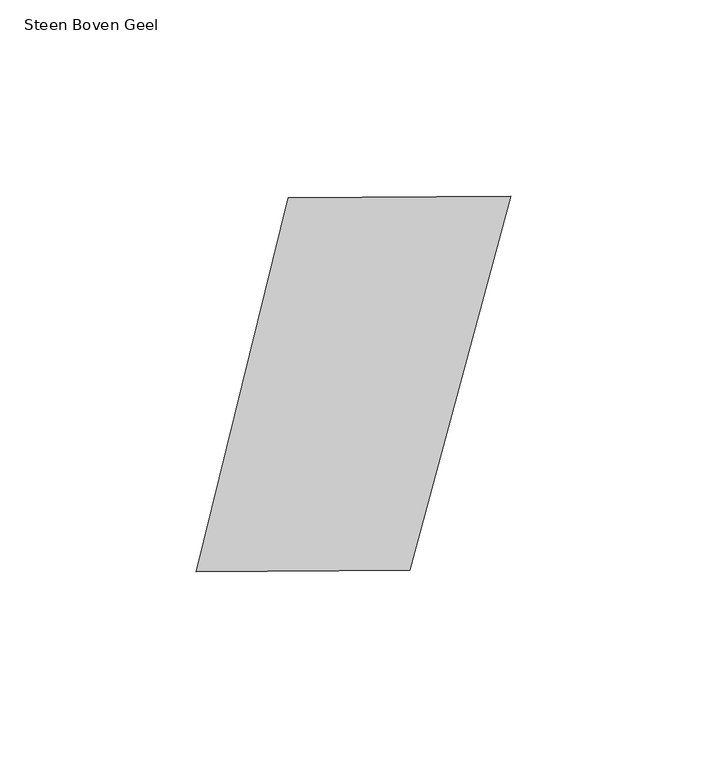
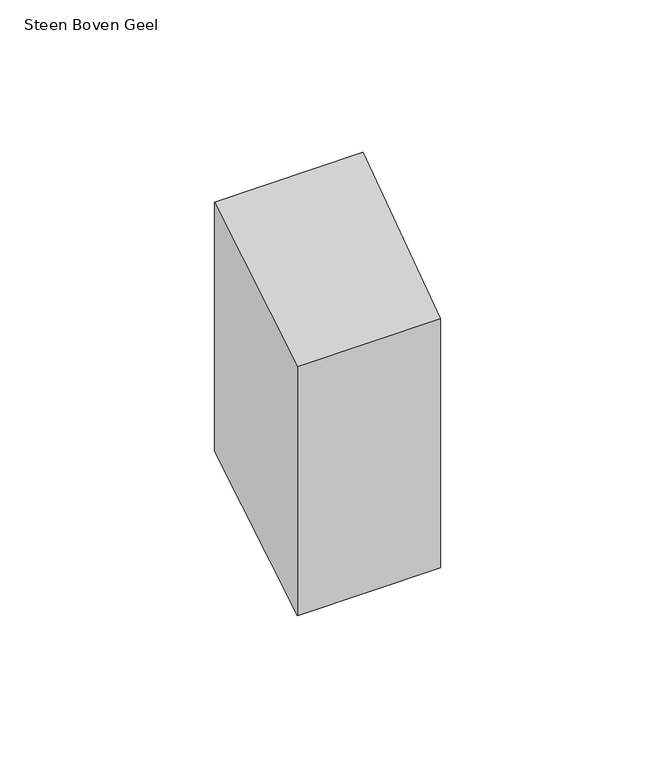
"""IFC4 building model written with IfcOpenShell, lengths in millimetres: proxy geometry, 00_GMA_steen_versie_4 : Steen Boven Geel."""

from ifc_helpers import new_model, si_unit, origin, origin_with_axes, place, context, project, spatial, polyline, outline, extrude, source, transform, mapped, element, save


def steen_boven_geel_e52851ac(model_context):
    return source(origin(), model_context, "Body", "SweptSolid", [
        extrude(outline(polyline([(114.0326098, 118.6673556), (88.372725, 23.2738668), (33.8296928, 22.8501526), (57.3678401, 118.2036955), (114.0326098, 118.6673556)])), origin_with_axes(), (0.0, 0.0, 1.0), 100.0),
    ])


if __name__ == "__main__":
    model = new_model("IFC4")
    model_context = context("Model", 3, world=origin())
    ifc_project = project(units=[si_unit("LENGTHUNIT", "METRE", prefix="MILLI")], contexts=[model_context])
    site = spatial("IfcSite", under=ifc_project)
    building = spatial("IfcBuilding", under=site)
    placement = place(None, origin())
    steen_boven_geel_shape = steen_boven_geel_e52851ac(model_context)
    element("IfcBuildingElementProxy", 1, Name="00_GMA_steen_versie_4 : Steen Boven Geel", ObjectType="00_GMA_steen_versie_4 : Steen Boven Geel", at=placement, inside=building, context=model_context, shape_type="MappedRepresentation", body=[
        mapped(steen_boven_geel_shape, transform((0.0, 0.0, 0.0), x_axis=(1.0, 0.0, 0.0), y_axis=(0.0, 1.0, 0.0), z_axis=(0.0, 0.0, 1.0))),
    ])
    save(model, "model.ifc")

# Revit data of these elements
# Type "00_GMA_steen_versie_4 : Steen Boven Geel"
#   StootVoegHalfBoven [instance default] = 5 mm
#   StootVoegHalf [instance default] = 5 mm
#   StootVoegBreedteOnder = 10 mm
#   StootVoegBreedteBoven = 10 mm
#   Steendikte = 100 mm
#   LintVoegOnderHalf = 5 mm
#   LintVoegOnder = 10 mm
#   LintVoegBovenHalf = 0 mm
#   LintVoegBoven = 0 mm
#   materiaal = 21_steen_geel
#   MateriaalVoeg = none
#   Default Elevation = 0
# Element 1 (IfcBuildingElementProxy, "00_GMA_steen_versie_4 : Steen Boven Geel")
#   Materials on its faces: "21_steen_geel"
# Materials
#   "21_steen_geel": class "Unassigned", colour RGB 202 202 0, transparency 0, Cost = 0
